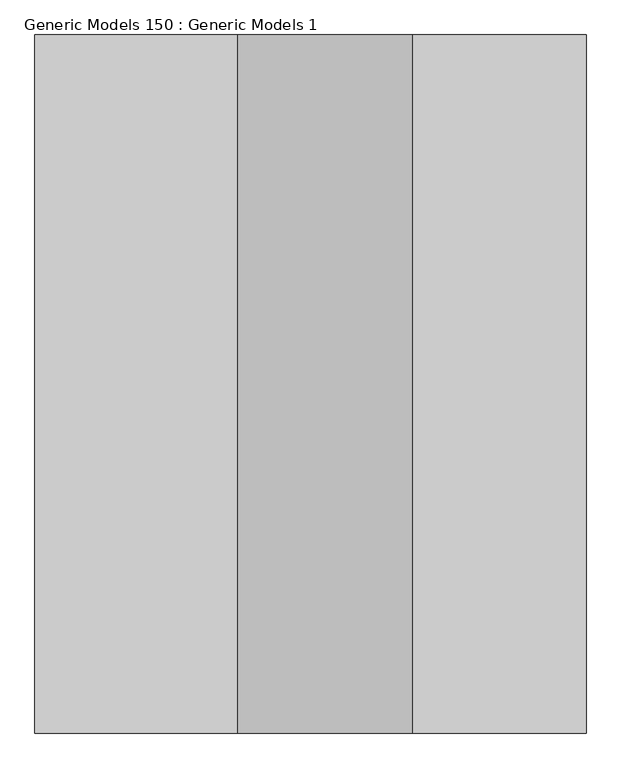
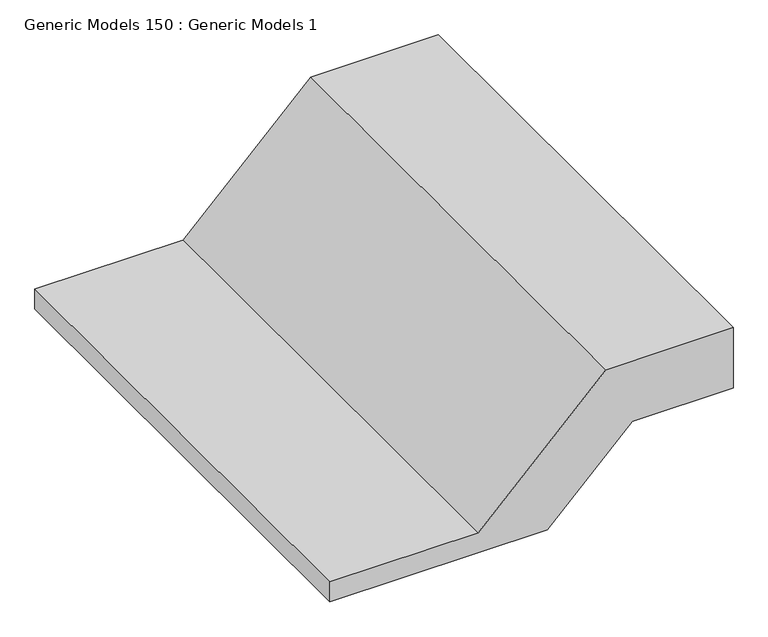
"""IFC4 building model written with IfcOpenShell, lengths in millimetres: proxy geometry, Generic Models 150 : Generic Models 1."""

from ifc_helpers import new_model, si_unit, frame, origin, place, context, project, spatial, polyline, outline, extrude, source, transform, mapped, element, save


def generic_models_150_generic_models_1_b2c8ea2b(model_context):
    return source(origin(), model_context, "Body", "SweptSolid", [
        extrude(outline(polyline([(-310.1710164, 52787.3395874), (-157.7710164, 52787.3395874), (-157.7710164, 52483.7302124), (-462.5710164, 52178.9302124), (-462.5710164, 51824.8420742), (-513.3710164, 51824.8420742), (-513.3710164, 52343.6563593), (-310.1710164, 52546.8563593), (-310.1710164, 52787.3395874)])), frame((0.0, 0.0, 0.0), z_axis=(0.0, 1.0, 0.0), x_axis=(0.0, 0.0, 1.0)), (0.0, 0.0, 1.0), 1219.2),
    ])


if __name__ == "__main__":
    model = new_model("IFC4")
    model_context = context("Model", 3, world=origin())
    ifc_project = project(units=[si_unit("LENGTHUNIT", "METRE", prefix="MILLI")], contexts=[model_context])
    site = spatial("IfcSite", under=ifc_project)
    building = spatial("IfcBuilding", under=site)
    placement = place(None, origin())
    generic_models_150_generic_models_1_shape = generic_models_150_generic_models_1_b2c8ea2b(model_context)
    element("IfcBuildingElementProxy", 1, Name="Generic Models 150 : Generic Models 1", ObjectType="Generic Models 150 : Generic Models 1", at=placement, inside=building, context=model_context, shape_type="MappedRepresentation", body=[
        mapped(generic_models_150_generic_models_1_shape, transform((0.0, 0.0, 0.0), x_axis=(1.0, 0.0, 0.0), y_axis=(0.0, 1.0, 0.0), z_axis=(0.0, 0.0, 1.0))),
    ])
    save(model, "model.ifc")

# Revit data of these elements
# Element 1 (IfcBuildingElementProxy, "Generic Models 150 : Generic Models 1")
#   Materials on its faces: "6\" COMPACTED CRUSHED STONE"
# Materials
#   "6\" COMPACTED CRUSHED STONE": class "Generic", colour RGB 255 255 255, transparency 0, Cost = 0
